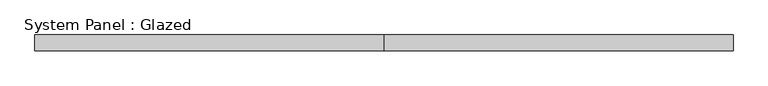
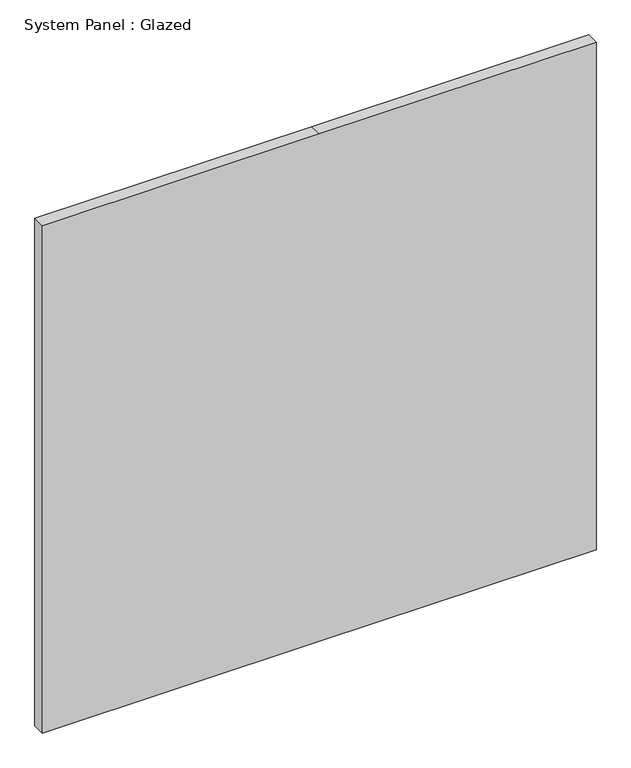
"""IFC4 building model written with IfcOpenShell, lengths in millimetres: plate geometry, System Panel : Glazed."""

from ifc_helpers import new_model, si_unit, frame, origin, place, context, project, spatial, polyline, outline, extrude, source, transform, mapped, element, save


def system_panel_glazed_eaf771f3(model_context):
    return source(origin(), model_context, "Body", "SweptSolid", [
        extrude(outline(polyline([(0.0, -1089.0), (0.0, 0.0), (0.0, 1089.0), (2110.0, 1089.0), (2110.0, 0.0), (2110.0, -1089.0), (0.0, -1089.0)])), frame((0.0, -25.0, 0.0), z_axis=(0.0, 1.0, 0.0), x_axis=(0.0, 0.0, 1.0)), (0.0, 0.0, 1.0), 50.0),
    ])


if __name__ == "__main__":
    model = new_model("IFC4")
    model_context = context("Model", 3, world=origin())
    ifc_project = project(units=[si_unit("LENGTHUNIT", "METRE", prefix="MILLI")], contexts=[model_context])
    site = spatial("IfcSite", under=ifc_project)
    building = spatial("IfcBuilding", under=site)
    placement = place(None, origin())
    system_panel_glazed_shape = system_panel_glazed_eaf771f3(model_context)
    element("IfcPlate", 1, ObjectType="System Panel : Glazed", at=placement, inside=building, context=model_context, shape_type="MappedRepresentation", body=[
        mapped(system_panel_glazed_shape, transform((0.0, 0.0, 0.0), x_axis=(1.0, 0.0, 0.0), y_axis=(0.0, 1.0, 0.0), z_axis=(0.0, 0.0, 1.0))),
    ])
    save(model, "model.ifc")

# Revit data of these elements
# Type "System Panel : Glazed"
#   Type Mark = "CW-GLASS"
# Element 1 (IfcPlate, "System Panel : Glazed")
#   Materials on its faces: "Glass_Clear"
# Materials
#   "Glass_Clear": class "Glass", colour RGB 128 128 255, transparency 0.8, Comments = "Rendering appearance not upgraded ", Cost = 0
